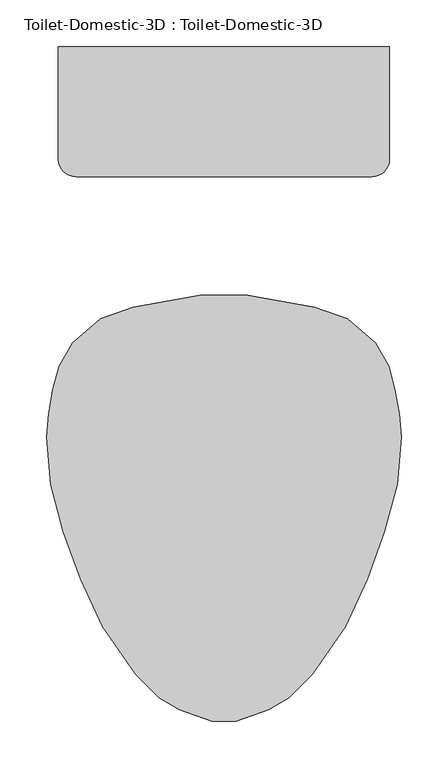
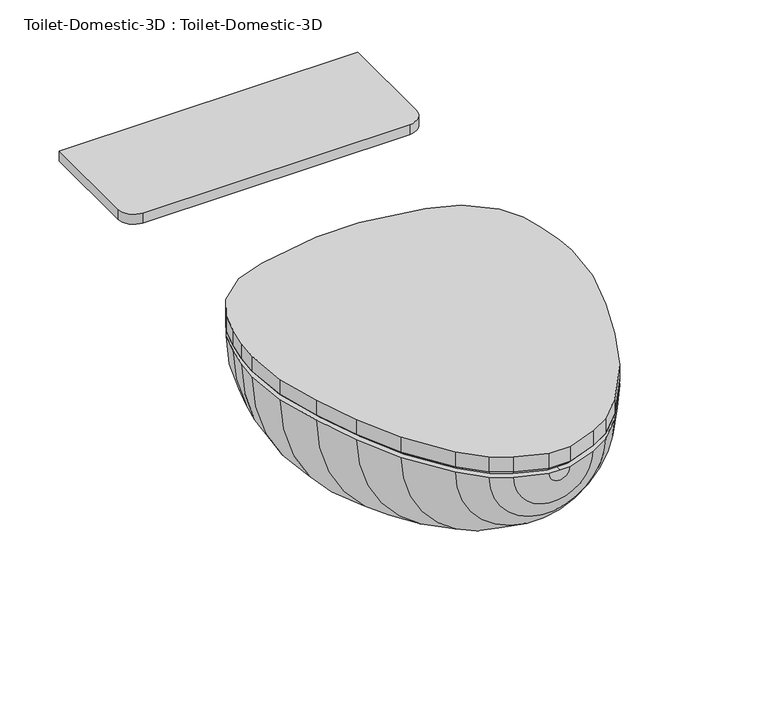
"""IFC4 building model written with IfcOpenShell, lengths in millimetres: flow terminal geometry, Toilet-Domestic-3D : Toilet-Domestic-3D."""

import ifcopenshell
import ifcopenshell.guid

model = None  # the IFC model being written
_history = None  # IfcOwnerHistory: only IFC2X3 demands one
_inside = {}  # id of a spatial element -> (the spatial element, [elements in it])
_under = {}  # id of a project, library or spatial element -> (it, [spatial elements below it])
_declared = {}  # id of a project -> (the project, [libraries it declares])
_typed = {}  # id of a type object -> (the type object, [elements of that type])
_made_of = {}  # id of a material, layer set ... -> (it, [elements and type objects made of it])


def new_model(schema):
    """Start an empty IFC model of exactly this schema.

    Asked for "IFC4X3", IfcOpenShell would pick the latest addendum, in which some entities
    have other attributes; the version numbers below select the first issue.
    IFC2X3 requires an IfcOwnerHistory on every rooted entity: one is made here for all.
    """
    global model, _history
    if schema == "IFC4X3":
        model = ifcopenshell.file(schema_version=(4, 3, 0, 0))
    else:
        model = ifcopenshell.file(schema=schema)
    _inside.clear()
    _under.clear()
    _declared.clear()
    _typed.clear()
    _made_of.clear()
    _history = None
    if model.schema == "IFC2X3":
        org = make("IfcOrganization", Name="unknown")
        user = make(
            "IfcPersonAndOrganization",
            ThePerson=make("IfcPerson", FamilyName="unknown"),
            TheOrganization=org,
        )
        app = make(
            "IfcApplication",
            ApplicationDeveloper=org,
            Version="unknown",
            ApplicationFullName="unknown",
            ApplicationIdentifier="unknown",
        )
        _history = make(
            "IfcOwnerHistory",
            OwningUser=user,
            OwningApplication=app,
            ChangeAction="ADDED",
            CreationDate=0,
        )
    return model


def make(cls, **values):
    """One entity of the class cls with the attributes given. An attribute that is None is left unset."""
    return model.create_entity(
        cls, **{name: value for name, value in values.items() if value is not None}
    )


def rooted(cls, **values):
    """An entity with a GlobalId (a new one), such as an element, a storey or a relation."""
    return make(cls, GlobalId=ifcopenshell.guid.new(), OwnerHistory=_history, **values)


def si_unit(unit_type, name, prefix=None):
    """IfcSIUnit, for example si_unit("LENGTHUNIT", "METRE", prefix="MILLI")."""
    return make("IfcSIUnit", UnitType=unit_type, Prefix=prefix, Name=name)


def assignment(units):
    """IfcUnitAssignment: the units of a project."""
    return None if units is None else make("IfcUnitAssignment", Units=units)


def point(xyz):
    """IfcCartesianPoint."""
    return None if xyz is None else make("IfcCartesianPoint", Coordinates=xyz)


def direction(xyz):
    """IfcDirection."""
    return None if xyz is None else make("IfcDirection", DirectionRatios=xyz)


def frame(location, z_axis=None, x_axis=None):
    """IfcAxis2Placement3D, a coordinate frame: its origin and axes. An axis left out is left unset."""
    return make(
        "IfcAxis2Placement3D",
        Location=point(location),
        Axis=direction(z_axis),
        RefDirection=direction(x_axis),
    )


def frame_2d(location, x_axis=None):
    """IfcAxis2Placement2D, a coordinate frame in the plane: its origin and x axis."""
    return make(
        "IfcAxis2Placement2D", Location=point(location), RefDirection=direction(x_axis)
    )


def origin():
    """The frame at (0, 0, 0) with its axes left unset."""
    return frame((0.0, 0.0, 0.0))


def place(relative_to, where):
    """IfcLocalPlacement: puts the frame where relative to a parent placement (None: the world)."""
    return make(
        "IfcLocalPlacement", PlacementRelTo=relative_to, RelativePlacement=where
    )


def context(
    kind, dimensions, precision=None, world=None, true_north=None, identifier=None
):
    """IfcGeometricRepresentationContext, for example the 3D "Model" context."""
    return make(
        "IfcGeometricRepresentationContext",
        ContextIdentifier=identifier,
        ContextType=kind,
        CoordinateSpaceDimension=dimensions,
        Precision=precision,
        WorldCoordinateSystem=world,
        TrueNorth=true_north,
    )


def project(units=None, contexts=None):
    """IfcProject with its units and contexts."""
    return rooted(
        "IfcProject",
        Name="project",
        RepresentationContexts=contexts,
        UnitsInContext=assignment(units),
    )


def spatial(cls, under=None, at=None, **own):
    """A site, building, storey or space (cls), placed at a placement, below another one or the project."""
    s = rooted(cls, ObjectPlacement=at, **own)
    if under is not None:
        _under.setdefault(under.id(), (under, []))[1].append(s)
    return s


def polyline(points):
    """IfcPolyline through the points."""
    return make("IfcPolyline", Points=[point(p) for p in points])


def circle_curve(where, radius):
    """IfcCircle in the frame where."""
    return make("IfcCircle", Position=where, Radius=radius)


def trimmed(basis, trim1, trim2, sense, master):
    """IfcTrimmedCurve: the piece of a basis curve between two trims."""
    return make(
        "IfcTrimmedCurve",
        BasisCurve=basis,
        Trim1=trim1,
        Trim2=trim2,
        SenseAgreement=sense,
        MasterRepresentation=master,
    )


def segment(curve, same_sense, transition):
    """IfcCompositeCurveSegment."""
    return make(
        "IfcCompositeCurveSegment",
        Transition=transition,
        SameSense=same_sense,
        ParentCurve=curve,
    )


def composite_curve(segments, self_intersect=None):
    """IfcCompositeCurve: segments joined end to end."""
    return make("IfcCompositeCurve", Segments=segments, SelfIntersect=self_intersect)


def outline(outer, holes=None, kind="AREA"):
    """IfcArbitraryClosedProfileDef: a profile drawn as a closed curve; with holes, ...WithVoids."""
    if holes is None:
        return make("IfcArbitraryClosedProfileDef", ProfileType=kind, OuterCurve=outer)
    return make(
        "IfcArbitraryProfileDefWithVoids",
        ProfileType=kind,
        OuterCurve=outer,
        InnerCurves=holes,
    )


def extrude(swept, where, along, depth):
    """IfcExtrudedAreaSolid: the profile swept, set in the frame where, extruded along a direction by depth."""
    return make(
        "IfcExtrudedAreaSolid",
        SweptArea=swept,
        Position=where,
        ExtrudedDirection=direction(along),
        Depth=depth,
    )


def faces_of(points, faces, orient=None, outer=None):
    """IfcFace entities. A face is a list of loops; a loop is a list of indices into points, from 0.

    orient and outer hold one flag for each loop. By default every Orientation is true, the
    first loop of a face is its IfcFaceOuterBound and the others are IfcFaceBound.
    """
    made = []
    for i, loops in enumerate(faces):
        bounds = []
        for j, loop in enumerate(loops):
            is_outer = j == 0 if outer is None else outer[i][j]
            bounds.append(
                make(
                    "IfcFaceOuterBound" if is_outer else "IfcFaceBound",
                    Bound=make("IfcPolyLoop", Polygon=[points[k] for k in loop]),
                    Orientation=True if orient is None else orient[i][j],
                )
            )
        made.append(make("IfcFace", Bounds=bounds))
    return made


def faceted_brep(points, faces, orient=None, outer=None, voids=None):
    """IfcFacetedBrep: a solid bounded by flat faces; with voids (closed shells), ...WithVoids."""
    shared = [point(p) for p in points]
    hull = make("IfcClosedShell", CfsFaces=faces_of(shared, faces, orient, outer))
    if voids is None:
        return make("IfcFacetedBrep", Outer=hull)
    return make(
        "IfcFacetedBrepWithVoids",
        Outer=hull,
        Voids=[
            make(cls, CfsFaces=faces_of(shared, fs, o, b)) for cls, fs, o, b in voids
        ],
    )


def shape(context_of_items, identifier, shape_type, items):
    """IfcShapeRepresentation: the items that make up one representation, for example the "Body"."""
    return make(
        "IfcShapeRepresentation",
        ContextOfItems=context_of_items,
        RepresentationIdentifier=identifier,
        RepresentationType=shape_type,
        Items=items,
    )


def source(mapping_origin, context_of_items, identifier, shape_type, items):
    """IfcRepresentationMap: a shape defined once, which mapped items show again and again."""
    return make(
        "IfcRepresentationMap",
        MappingOrigin=mapping_origin,
        MappedRepresentation=shape(context_of_items, identifier, shape_type, items),
    )


def transform(
    local_origin,
    x_axis=None,
    y_axis=None,
    z_axis=None,
    scale=None,
    scale2=None,
    scale3=None,
    uniform=True,
):
    """IfcCartesianTransformationOperator3D, or its non-uniform kind. x_axis, y_axis, z_axis: its Axis1, 2, 3."""
    if uniform:
        return make(
            "IfcCartesianTransformationOperator3D",
            Axis1=direction(x_axis),
            Axis2=direction(y_axis),
            LocalOrigin=point(local_origin),
            Scale=scale,
            Axis3=direction(z_axis),
        )
    return make(
        "IfcCartesianTransformationOperator3DnonUniform",
        Axis1=direction(x_axis),
        Axis2=direction(y_axis),
        LocalOrigin=point(local_origin),
        Scale=scale,
        Axis3=direction(z_axis),
        Scale2=scale2,
        Scale3=scale3,
    )


def mapped(mapping_source, mapping_target):
    """IfcMappedItem: shows the shape of a source again, moved by a transform."""
    return make(
        "IfcMappedItem", MappingSource=mapping_source, MappingTarget=mapping_target
    )


def made_of(thing, what):
    """Note that an element or type object is made of a material, layer set ...; save() writes the relation."""
    if what is not None:
        _made_of.setdefault(what.id(), (what, []))[1].append(thing)
    return thing


def element(
    cls,
    number,
    at=None,
    inside=None,
    cuts=None,
    type_object=None,
    material=None,
    context=None,
    identifier="Body",
    shape_type=None,
    held_by="IfcProductDefinitionShape",
    body=None,
    shapes=None,
    **own,
):
    """One element of the class cls, such as IfcWall. Its Tag is "e" and its number.

    at: its placement. inside: the storey or other place that contains it. cuts: it is an
    opening in that element (IfcRelVoidsElement). A single representation is given by context,
    identifier, shape_type and body (its items); several are given by shapes. held_by: the class
    of the entity that holds the representations. save() writes the other relations.
    """
    e = rooted(cls, Tag="e%d" % number, ObjectPlacement=at, **own)
    if body is not None:
        shapes = [shape(context, identifier, shape_type, body)]
    if shapes is not None:
        e.Representation = make(held_by, Representations=shapes)
    if inside is not None:
        _inside.setdefault(inside.id(), (inside, []))[1].append(e)
    if cuts is not None:
        rooted(
            "IfcRelVoidsElement", RelatingBuildingElement=cuts, RelatedOpeningElement=e
        )
    if type_object is not None:
        _typed.setdefault(type_object.id(), (type_object, []))[1].append(e)
    return made_of(e, material)


def aggregate(whole, parts):
    """IfcRelAggregates: a whole, such as a stair, and the parts it consists of."""
    return rooted("IfcRelAggregates", RelatingObject=whole, RelatedObjects=parts)


def save(model, path):
    """Write the relations noted so far, then the file.

    IfcRelAggregates (storeys below a building ...), IfcRelContainedInSpatialStructure (elements
    in a storey), IfcRelDefinesByType, IfcRelAssociatesMaterial and IfcRelDeclares: one each for
    every whole, place, type object, material and project.
    """
    for whole, parts in _under.values():
        aggregate(whole, parts)
    for where, things in _inside.values():
        rooted(
            "IfcRelContainedInSpatialStructure",
            RelatedElements=things,
            RelatingStructure=where,
        )
    for kind, things in _typed.values():
        rooted("IfcRelDefinesByType", RelatedObjects=things, RelatingType=kind)
    for what, things in _made_of.values():
        rooted("IfcRelAssociatesMaterial", RelatedObjects=things, RelatingMaterial=what)
    for by, libraries in _declared.values():
        rooted("IfcRelDeclares", RelatingContext=by, RelatedDefinitions=libraries)
    model.write(path)


def plane_surface(at):
    """IfcPlane: the flat surface through the origin of the frame at, square to its z axis."""
    return make("IfcPlane", Position=at)


def revolved_surface(curve, axis_point, axis_direction):
    """IfcSurfaceOfRevolution: the curve turned about the line through axis_point along axis_direction."""
    return make(
        "IfcSurfaceOfRevolution",
        SweptCurve=make("IfcArbitraryOpenProfileDef", ProfileType="CURVE", Curve=curve),
        AxisPosition=make("IfcAxis1Placement", Location=point(axis_point), Axis=direction(axis_direction)),
    )


def advanced_brep(points, edges, surfaces, faces):
    """IfcAdvancedBrep: a solid bounded by faces that lie on surfaces and meet in shared edges.

    An edge is (start, end): straight between two places in points (the first is 0);
    or (start, end, curve); or (start, end, curve, False) where it runs against its curve.
    A face is (place in surfaces, loops), or (place, loops, False) where it looks against
    its surface's normal. A loop lists edges by number (the first is 1), with a minus sign
    where the edge is run from its end to its start. The first loop is the outer one.
    """
    corners = [point(p) for p in points]
    vertices = [make("IfcVertexPoint", VertexGeometry=c) for c in corners]
    made = []
    for start, end, *more in edges:
        made.append(
            make(
                "IfcEdgeCurve",
                EdgeStart=vertices[start],
                EdgeEnd=vertices[end],
                EdgeGeometry=more[0] if more else make("IfcPolyline", Points=[corners[start], corners[end]]),
                SameSense=more[1] if len(more) > 1 else True,
            )
        )
    hull = []
    for where, loops, *sense in faces:
        bounds = []
        for j, loop in enumerate(loops):
            ring = [make("IfcOrientedEdge", EdgeElement=made[abs(k) - 1], Orientation=k > 0) for k in loop]
            bounds.append(
                make(
                    "IfcFaceOuterBound" if j == 0 else "IfcFaceBound",
                    Bound=make("IfcEdgeLoop", EdgeList=ring),
                    Orientation=True,
                )
            )
        hull.append(make("IfcAdvancedFace", Bounds=bounds, FaceSurface=surfaces[where], SameSense=sense[0] if sense else True))
    return make("IfcAdvancedBrep", Outer=make("IfcClosedShell", CfsFaces=hull))


def toilet_domestic_3d_toilet_domestic_3d_183bbd19(model_context):
    return source(origin(), model_context, "Body", "SolidModel", [
        advanced_brep(
        [(-25.4, 152.4, 361.95), (-97.4252791, 139.7, 361.95), (-132.3182423, 127.0, 361.95), (-162.5887836, 101.6, 361.95), (-176.9845865, 76.2, 361.95), (-183.790496, 50.8, 361.95), (-188.2862441, 25.3033453, 361.95), (-190.5, 0.0, 361.95), (-186.0724883, -50.6066907, 361.95), (-172.4088722, -101.6, 361.95), (-153.9191843, -152.4, 361.95), (-130.2307553, -203.2, 361.95), (-94.9900085, -254.0, 361.95), (-69.5900085, -279.4, 361.95), (-47.5929632, -292.1, 361.95), (-12.7, -304.8, 361.95), (0.0, -304.8, 361.95), (0.0, -284.592034, 361.95), (-12.5224565, -284.592034, 361.95), (-39.5113323, -274.7688865, 361.95), (-58.4178985, -263.8531754, 361.95), (-79.2146703, -243.0564036, 361.95), (-114.0255101, -192.8761202, 361.95), (-136.654021, -144.3491221, 361.95), (-154.575847, -95.1093097, 361.95), (-167.7238545, -46.0402777, 361.95), (-171.5645445, -2.1409906, 361.95), (-169.3087351, 23.6430284, 361.95), (-165.101298, 47.5045901, 361.95), (-159.5484355, 68.2281551, 361.95), (-146.1085923, 90.5605136, 361.95), (-121.9980886, 110.7916284, 361.95), (-94.1172813, 120.9394123, 361.95), (-22.0920022, 133.6394123, 361.95), (0.0, 133.6394123, 361.95), (0.0, 152.4, 361.95), (25.4, 152.4, 361.95), (22.0920022, 133.6394123, 361.95), (94.1172813, 120.9394123, 361.95), (121.9980886, 110.7916284, 361.95), (146.1085923, 90.5605136, 361.95), (159.5484355, 68.2281551, 361.95), (165.101298, 47.5045901, 361.95), (169.3087351, 23.6430284, 361.95), (171.5645445, -2.1409906, 361.95), (167.7238545, -46.0402777, 361.95), (154.575847, -95.1093097, 361.95), (136.654021, -144.3491221, 361.95), (114.0255101, -192.8761202, 361.95), (79.2146703, -243.0564036, 361.95), (58.4178985, -263.8531754, 361.95), (39.5113323, -274.7688865, 361.95), (12.5224565, -284.592034, 361.95), (12.7, -304.8, 361.95), (47.5929632, -292.1, 361.95), (69.5900085, -279.4, 361.95), (94.9900085, -254.0, 361.95), (130.2307553, -203.2, 361.95), (153.9191843, -152.4, 361.95), (172.4088722, -101.6, 361.95), (186.0724883, -50.6066907, 361.95), (190.5, 0.0, 361.95), (188.2862441, 25.3033453, 361.95), (183.790496, 50.8, 361.95), (176.9845865, 76.2, 361.95), (162.5887836, 101.6, 361.95), (132.3182423, 127.0, 361.95), (97.4252791, 139.7, 361.95)],
        [
            (0, 1),
            (1, 2),
            (2, 3),
            (3, 4),
            (4, 5),
            (5, 6),
            (6, 7),
            (7, 8),
            (8, 9),
            (9, 10),
            (10, 11),
            (11, 12),
            (12, 13),
            (13, 14),
            (14, 15),
            (15, 16),
            (16, 17),
            (17, 18),
            (18, 19),
            (19, 20),
            (20, 21),
            (21, 22),
            (22, 23),
            (23, 24),
            (24, 25),
            (25, 26),
            (26, 27),
            (27, 28),
            (28, 29),
            (29, 30),
            (30, 31),
            (31, 32),
            (32, 33),
            (33, 34),
            (34, 35),
            (35, 0),
            (36, 35),
            (34, 37),
            (37, 38),
            (38, 39),
            (39, 40),
            (40, 41),
            (41, 42),
            (42, 43),
            (43, 44),
            (44, 45),
            (45, 46),
            (46, 47),
            (47, 48),
            (48, 49),
            (49, 50),
            (50, 51),
            (51, 52),
            (52, 17),
            (16, 53),
            (53, 54),
            (54, 55),
            (55, 56),
            (56, 57),
            (57, 58),
            (58, 59),
            (59, 60),
            (60, 61),
            (61, 62),
            (62, 63),
            (63, 64),
            (64, 65),
            (65, 66),
            (66, 67),
            (67, 36),
            (67, 1, circle_curve(frame((0.0, 139.7, 361.95), z_axis=(0.0, 1.0, 0.0), x_axis=(-1.0, 0.0, 0.0)), 97.4252791)),
            (0, 36, circle_curve(frame((0.0, 152.4, 361.95), z_axis=(0.0, -1.0, 0.0), x_axis=(-1.0, 0.0, 0.0)), 25.4)),
            (66, 2, circle_curve(frame((0.0, 127.0, 361.95), z_axis=(0.0, 1.0, 0.0), x_axis=(-1.0, 0.0, 0.0)), 132.3182423)),
            (65, 3, circle_curve(frame((0.0, 101.6, 361.95), z_axis=(0.0, 1.0, 0.0), x_axis=(-1.0, 0.0, 0.0)), 162.5887836)),
            (64, 4, circle_curve(frame((0.0, 76.2, 361.95), z_axis=(0.0, 1.0, 0.0), x_axis=(-1.0, 0.0, 0.0)), 176.9845865)),
            (63, 5, circle_curve(frame((0.0, 50.8, 361.95), z_axis=(0.0, 1.0, 0.0), x_axis=(-1.0, 0.0, 0.0)), 183.790496)),
            (62, 6, circle_curve(frame((0.0, 25.3033453, 361.95), z_axis=(0.0, 1.0, 0.0), x_axis=(-1.0, 0.0, 0.0)), 188.2862441)),
            (61, 7, circle_curve(frame((0.0, 0.0, 361.95), z_axis=(0.0, 1.0, 0.0), x_axis=(-1.0, 0.0, 0.0)), 190.5)),
            (60, 8, circle_curve(frame((0.0, -50.6066907, 361.95), z_axis=(0.0, 1.0, 0.0), x_axis=(-1.0, 0.0, 0.0)), 186.0724883)),
            (59, 9, circle_curve(frame((0.0, -101.6, 361.95), z_axis=(0.0, 1.0, 0.0), x_axis=(-1.0, 0.0, 0.0)), 172.4088722)),
            (58, 10, circle_curve(frame((0.0, -152.4, 361.95), z_axis=(0.0, 1.0, 0.0), x_axis=(-1.0, 0.0, 0.0)), 153.9191843)),
            (57, 11, circle_curve(frame((0.0, -203.2, 361.95), z_axis=(0.0, 1.0, 0.0), x_axis=(-1.0, 0.0, 0.0)), 130.2307553)),
            (56, 12, circle_curve(frame((0.0, -254.0, 361.95), z_axis=(0.0, 1.0, 0.0), x_axis=(-1.0, 0.0, 0.0)), 94.9900085)),
            (55, 13, circle_curve(frame((0.0, -279.4, 361.95), z_axis=(0.0, 1.0, 0.0), x_axis=(-1.0, 0.0, 0.0)), 69.5900085)),
            (54, 14, circle_curve(frame((0.0, -292.1, 361.95), z_axis=(0.0, 1.0, 0.0), x_axis=(-1.0, 0.0, 0.0)), 47.5929632)),
            (53, 15, circle_curve(frame((0.0, -304.8, 361.95), z_axis=(0.0, 1.0, 0.0), x_axis=(-1.0, 0.0, 0.0)), 12.7)),
            (52, 18, circle_curve(frame((0.0, -284.592034, 361.95), z_axis=(0.0, 1.0, 0.0), x_axis=(-1.0, 0.0, 0.0)), 12.5224565)),
            (51, 19, circle_curve(frame((0.0, -274.7688865, 361.95), z_axis=(0.0, 1.0, 0.0), x_axis=(-1.0, 0.0, 0.0)), 39.5113323)),
            (50, 20, circle_curve(frame((0.0, -263.8531754, 361.95), z_axis=(0.0, 1.0, 0.0), x_axis=(-1.0, 0.0, 0.0)), 58.4178985)),
            (49, 21, circle_curve(frame((0.0, -243.0564036, 361.95), z_axis=(0.0, 1.0, 0.0), x_axis=(-1.0, 0.0, 0.0)), 79.2146703)),
            (48, 22, circle_curve(frame((0.0, -192.8761202, 361.95), z_axis=(0.0, 1.0, 0.0), x_axis=(-1.0, 0.0, 0.0)), 114.0255101)),
            (47, 23, circle_curve(frame((0.0, -144.3491221, 361.95), z_axis=(0.0, 1.0, 0.0), x_axis=(-1.0, 0.0, 0.0)), 136.654021)),
            (46, 24, circle_curve(frame((0.0, -95.1093097, 361.95), z_axis=(0.0, 1.0, 0.0), x_axis=(-1.0, 0.0, 0.0)), 154.575847)),
            (45, 25, circle_curve(frame((0.0, -46.0402777, 361.95), z_axis=(0.0, 1.0, 0.0), x_axis=(-1.0, 0.0, 0.0)), 167.7238545)),
            (44, 26, circle_curve(frame((0.0, -2.1409906, 361.95), z_axis=(0.0, 1.0, 0.0), x_axis=(-1.0, 0.0, 0.0)), 171.5645445)),
            (43, 27, circle_curve(frame((0.0, 23.6430284, 361.95), z_axis=(0.0, 1.0, 0.0), x_axis=(-1.0, 0.0, 0.0)), 169.3087351)),
            (42, 28, circle_curve(frame((0.0, 47.5045901, 361.95), z_axis=(0.0, 1.0, 0.0), x_axis=(-1.0, 0.0, 0.0)), 165.101298)),
            (41, 29, circle_curve(frame((0.0, 68.2281551, 361.95), z_axis=(0.0, 1.0, 0.0), x_axis=(-1.0, 0.0, 0.0)), 159.5484355)),
            (40, 30, circle_curve(frame((0.0, 90.5605136, 361.95), z_axis=(0.0, 1.0, 0.0), x_axis=(-1.0, 0.0, 0.0)), 146.1085923)),
            (39, 31, circle_curve(frame((0.0, 110.7916284, 361.95), z_axis=(0.0, 1.0, 0.0), x_axis=(-1.0, 0.0, 0.0)), 121.9980886)),
            (38, 32, circle_curve(frame((0.0, 120.9394123, 361.95), z_axis=(0.0, 1.0, 0.0), x_axis=(-1.0, 0.0, 0.0)), 94.1172813)),
            (37, 33, circle_curve(frame((0.0, 133.6394123, 361.95), z_axis=(0.0, 1.0, 0.0), x_axis=(-1.0, 0.0, 0.0)), 22.0920022)),
        ],
        [
            plane_surface(frame((0.0, 175.1599017, 361.95), z_axis=(0.0, 0.0, 1.0), x_axis=(-1.0, 0.0, 0.0))),
            plane_surface(frame((0.0, 175.1599017, 361.95), z_axis=(0.0, 0.0, 1.0), x_axis=(1.0, 0.0, 0.0))),
            revolved_surface(polyline([(-25.4, 152.4, 361.95), (-97.4252791, 139.7, 361.95)]), (0.0, 175.1599017, 361.95), (0.0, -1.0, 0.0)),
            revolved_surface(polyline([(-97.4252791, 139.7, 361.95), (-132.3182423, 127.0, 361.95)]), (0.0, 175.1599017, 361.95), (0.0, -1.0, 0.0)),
            revolved_surface(polyline([(-132.3182423, 127.0, 361.95), (-162.5887836, 101.6, 361.95)]), (0.0, 175.1599017, 361.95), (0.0, -1.0, 0.0)),
            revolved_surface(polyline([(-162.5887836, 101.6, 361.95), (-176.9845865, 76.2, 361.95)]), (0.0, 175.1599017, 361.95), (0.0, -1.0, 0.0)),
            revolved_surface(polyline([(-176.9845865, 76.2, 361.95), (-183.790496, 50.8, 361.95)]), (0.0, 175.1599017, 361.95), (0.0, -1.0, 0.0)),
            revolved_surface(polyline([(-183.790496, 50.8, 361.95), (-188.2862441, 25.3033453, 361.95)]), (0.0, 175.1599017, 361.95), (0.0, -1.0, 0.0)),
            revolved_surface(polyline([(-188.2862441, 25.3033453, 361.95), (-190.5, 0.0, 361.95)]), (0.0, 175.1599017, 361.95), (0.0, -1.0, 0.0)),
            revolved_surface(polyline([(-190.5, 0.0, 361.95), (-186.0724883, -50.6066907, 361.95)]), (0.0, 175.1599017, 361.95), (0.0, -1.0, 0.0)),
            revolved_surface(polyline([(-186.0724883, -50.6066907, 361.95), (-172.4088722, -101.6, 361.95)]), (0.0, 175.1599017, 361.95), (0.0, -1.0, 0.0)),
            revolved_surface(polyline([(-172.4088722, -101.6, 361.95), (-153.9191843, -152.4, 361.95)]), (0.0, 175.1599017, 361.95), (0.0, -1.0, 0.0)),
            revolved_surface(polyline([(-153.9191843, -152.4, 361.95), (-130.2307553, -203.2, 361.95)]), (0.0, 175.1599017, 361.95), (0.0, -1.0, 0.0)),
            revolved_surface(polyline([(-130.2307553, -203.2, 361.95), (-94.9900085, -254.0, 361.95)]), (0.0, 175.1599017, 361.95), (0.0, -1.0, 0.0)),
            revolved_surface(polyline([(-94.9900085, -254.0, 361.95), (-69.5900085, -279.4, 361.95)]), (0.0, 175.1599017, 361.95), (0.0, -1.0, 0.0)),
            revolved_surface(polyline([(-69.5900085, -279.4, 361.95), (-47.5929632, -292.1, 361.95)]), (0.0, 175.1599017, 361.95), (0.0, -1.0, 0.0)),
            revolved_surface(polyline([(-47.5929632, -292.1, 361.95), (-12.7, -304.8, 361.95)]), (0.0, 175.1599017, 361.95), (0.0, -1.0, 0.0)),
            plane_surface(frame((0.0, -304.8, 361.95), z_axis=(0.0, -1.0, 0.0), x_axis=(-1.0, 0.0, 0.0))),
            plane_surface(frame((0.0, -284.592034, 361.95), z_axis=(0.0, 1.0, 0.0), x_axis=(-1.0, 0.0, 0.0))),
            revolved_surface(polyline([(-12.5224565, -284.592034, 361.95), (-39.5113323, -274.7688865, 361.95)]), (0.0, 175.1599017, 361.95), (0.0, -1.0, 0.0)),
            revolved_surface(polyline([(-39.5113323, -274.7688865, 361.95), (-58.4178985, -263.8531754, 361.95)]), (0.0, 175.1599017, 361.95), (0.0, -1.0, 0.0)),
            revolved_surface(polyline([(-58.4178985, -263.8531754, 361.95), (-79.2146703, -243.0564036, 361.95)]), (0.0, 175.1599017, 361.95), (0.0, -1.0, 0.0)),
            revolved_surface(polyline([(-79.2146703, -243.0564036, 361.95), (-114.0255101, -192.8761202, 361.95)]), (0.0, 175.1599017, 361.95), (0.0, -1.0, 0.0)),
            revolved_surface(polyline([(-114.0255101, -192.8761202, 361.95), (-136.654021, -144.3491221, 361.95)]), (0.0, 175.1599017, 361.95), (0.0, -1.0, 0.0)),
            revolved_surface(polyline([(-136.654021, -144.3491221, 361.95), (-154.575847, -95.1093097, 361.95)]), (0.0, 175.1599017, 361.95), (0.0, -1.0, 0.0)),
            revolved_surface(polyline([(-154.575847, -95.1093097, 361.95), (-167.7238545, -46.0402777, 361.95)]), (0.0, 175.1599017, 361.95), (0.0, -1.0, 0.0)),
            revolved_surface(polyline([(-167.7238545, -46.0402777, 361.95), (-171.5645445, -2.1409906, 361.95)]), (0.0, 175.1599017, 361.95), (0.0, -1.0, 0.0)),
            revolved_surface(polyline([(-171.5645445, -2.1409906, 361.95), (-169.3087351, 23.6430284, 361.95)]), (0.0, 175.1599017, 361.95), (0.0, -1.0, 0.0)),
            revolved_surface(polyline([(-169.3087351, 23.6430284, 361.95), (-165.101298, 47.5045901, 361.95)]), (0.0, 175.1599017, 361.95), (0.0, -1.0, 0.0)),
            revolved_surface(polyline([(-165.101298, 47.5045901, 361.95), (-159.5484355, 68.2281551, 361.95)]), (0.0, 175.1599017, 361.95), (0.0, -1.0, 0.0)),
            revolved_surface(polyline([(-159.5484355, 68.2281551, 361.95), (-146.1085923, 90.5605136, 361.95)]), (0.0, 175.1599017, 361.95), (0.0, -1.0, 0.0)),
            revolved_surface(polyline([(-146.1085923, 90.5605136, 361.95), (-121.9980886, 110.7916284, 361.95)]), (0.0, 175.1599017, 361.95), (0.0, -1.0, 0.0)),
            revolved_surface(polyline([(-121.9980886, 110.7916284, 361.95), (-94.1172813, 120.9394123, 361.95)]), (0.0, 175.1599017, 361.95), (0.0, -1.0, 0.0)),
            revolved_surface(polyline([(-94.1172813, 120.9394123, 361.95), (-22.0920022, 133.6394123, 361.95)]), (0.0, 175.1599017, 361.95), (0.0, -1.0, 0.0)),
            plane_surface(frame((0.0, 133.6394123, 361.95), z_axis=(0.0, -1.0, 0.0), x_axis=(-1.0, 0.0, 0.0))),
            plane_surface(frame((0.0, 152.4, 361.95), z_axis=(0.0, 1.0, 0.0), x_axis=(-1.0, 0.0, 0.0))),
        ],
        [
            (0, [[1, 2, 3, 4, 5, 6, 7, 8, 9, 10, 11, 12, 13, 14, 15, 16, 17, 18, 19, 20, 21, 22, 23, 24, 25, 26, 27, 28, 29, 30, 31, 32, 33, 34, 35, 36]]),
            (1, [[37, -35, 38, 39, 40, 41, 42, 43, 44, 45, 46, 47, 48, 49, 50, 51, 52, 53, 54, -17, 55, 56, 57, 58, 59, 60, 61, 62, 63, 64, 65, 66, 67, 68, 69, 70]]),
            (2, [[71, -1, 72, -70]]),
            (3, [[73, -2, -71, -69]]),
            (4, [[74, -3, -73, -68]]),
            (5, [[75, -4, -74, -67]]),
            (6, [[76, -5, -75, -66]]),
            (7, [[77, -6, -76, -65]]),
            (8, [[78, -7, -77, -64]]),
            (9, [[79, -8, -78, -63]]),
            (10, [[80, -9, -79, -62]]),
            (11, [[81, -10, -80, -61]]),
            (12, [[82, -11, -81, -60]]),
            (13, [[83, -12, -82, -59]]),
            (14, [[84, -13, -83, -58]]),
            (15, [[85, -14, -84, -57]]),
            (16, [[86, -15, -85, -56]]),
            (17, [[-16, -86, -55]]),
            (18, [[87, -18, -54]]),
            (19, [[88, -19, -87, -53]]),
            (20, [[89, -20, -88, -52]]),
            (21, [[90, -21, -89, -51]]),
            (22, [[91, -22, -90, -50]]),
            (23, [[92, -23, -91, -49]]),
            (24, [[93, -24, -92, -48]]),
            (25, [[94, -25, -93, -47]]),
            (26, [[95, -26, -94, -46]]),
            (27, [[96, -27, -95, -45]]),
            (28, [[97, -28, -96, -44]]),
            (29, [[98, -29, -97, -43]]),
            (30, [[99, -30, -98, -42]]),
            (31, [[100, -31, -99, -41]]),
            (32, [[101, -32, -100, -40]]),
            (33, [[102, -33, -101, -39]]),
            (34, [[-34, -102, -38]]),
            (35, [[-72, -36, -37]]),
        ],
    ),
        faceted_brep([(-97.4252791, 139.7, 368.3), (-132.3182423, 127.0, 368.3), (-162.5887836, 101.6, 368.3), (-176.9845865, 76.2, 368.3), (-183.790496, 50.8, 368.3), (-188.2862441, 25.3033453, 368.3), (-190.5, 0.0, 368.3), (-186.0724883, -50.6066907, 368.3), (-172.4088722, -101.6, 368.3), (-153.9191843, -152.4, 368.3), (-130.2307553, -203.2, 368.3), (-94.9900085, -254.0, 368.3), (-69.5900085, -279.4, 368.3), (-47.5929632, -292.1, 368.3), (-12.7, -304.8, 368.3), (12.7, -304.8, 368.3), (47.5929632, -292.1, 368.3), (69.5900085, -279.4, 368.3), (94.9900085, -254.0, 368.3), (130.2307553, -203.2, 368.3), (153.9191843, -152.4, 368.3), (172.4088722, -101.6, 368.3), (186.0724883, -50.6066907, 368.3), (190.5, 0.0, 368.3), (188.2862441, 25.3033453, 368.3), (183.790496, 50.8, 368.3), (176.9845865, 76.2, 368.3), (162.5887836, 101.6, 368.3), (132.3182423, 127.0, 368.3), (97.4252791, 139.7, 368.3), (25.4, 152.4, 368.3), (-25.4, 152.4, 368.3), (-95.7755003, 133.5429415, 361.95), (-24.844447, 146.05, 361.95), (24.844447, 146.05, 361.95), (95.7755003, 133.5429415, 361.95), (129.0942628, 121.4159037, 361.95), (157.6293435, 97.472128, 361.95), (171.060664, 73.773864, 361.95), (177.5851102, 49.4242991, 361.95), (181.9845715, 24.4737144, 361.95), (184.125744, 0.0, 361.95), (179.7950716, -49.4998127, 361.95), (166.347, -99.688699, 361.95), (148.0469602, -149.9676451, 361.95), (124.7045808, -200.0255393, 361.95), (90.0971582, -249.9125941, 361.95), (65.691017, -274.3187354, 361.95), (44.8990862, -286.3229622, 361.95), (11.5803237, -298.45, 361.95), (-11.5803237, -298.45, 361.95), (-44.8990862, -286.3229622, 361.95), (-65.691017, -274.3187354, 361.95), (-90.0971582, -249.9125941, 361.95), (-124.7045808, -200.0255393, 361.95), (-148.0469602, -149.9676451, 361.95), (-166.347, -99.688699, 361.95), (-179.7950716, -49.4998127, 361.95), (-184.125744, 0.0, 361.95), (-181.9845715, 24.4737144, 361.95), (-177.5851102, 49.4242991, 361.95), (-171.060664, 73.773864, 361.95), (-157.6293435, 97.472128, 361.95), (-129.0942628, 121.4159037, 361.95)], [[[0, 1, 2, 3, 4, 5, 6, 7, 8, 9, 10, 11, 12, 13, 14, 15, 16, 17, 18, 19, 20, 21, 22, 23, 24, 25, 26, 27, 28, 29, 30, 31]], [[32, 33, 34, 35, 36, 37, 38, 39, 40, 41, 42, 43, 44, 45, 46, 47, 48, 49, 50, 51, 52, 53, 54, 55, 56, 57, 58, 59, 60, 61, 62, 63]], [[32, 63, 1, 0]], [[63, 62, 2, 1]], [[62, 61, 3, 2]], [[61, 60, 4, 3]], [[60, 59, 5, 4]], [[59, 58, 6, 5]], [[58, 57, 7, 6]], [[57, 56, 8, 7]], [[56, 55, 9, 8]], [[55, 54, 10, 9]], [[54, 53, 11, 10]], [[53, 52, 12, 11]], [[52, 51, 13, 12]], [[51, 50, 14, 13]], [[50, 49, 15, 14]], [[49, 48, 16, 15]], [[48, 47, 17, 16]], [[47, 46, 18, 17]], [[46, 45, 19, 18]], [[45, 44, 20, 19]], [[44, 43, 21, 20]], [[43, 42, 22, 21]], [[42, 41, 23, 22]], [[41, 40, 24, 23]], [[40, 39, 25, 24]], [[39, 38, 26, 25]], [[38, 37, 27, 26]], [[37, 36, 28, 27]], [[36, 35, 29, 28]], [[35, 34, 30, 29]], [[34, 33, 31, 30]], [[33, 32, 0, 31]]]),
        extrude(outline(composite_curve([segment(polyline([(177.8, 419.1), (177.8, 298.45)]), True, "CONTINUOUS"), segment(trimmed(circle_curve(frame_2d((158.75, 298.45)), 19.05), [point((177.8, 298.45))], [point((158.75, 279.4))], False, "CARTESIAN"), True, "CONTINUOUS"), segment(polyline([(158.75, 279.4), (-158.75, 279.4)]), True, "CONTINUOUS"), segment(trimmed(circle_curve(frame_2d((-158.75, 298.45)), 19.05), [point((-158.75, 279.4))], [point((-177.8, 298.45))], False, "CARTESIAN"), True, "CONTINUOUS"), segment(polyline([(-177.8, 298.45), (-177.8, 419.1), (177.8, 419.1)]), True, "CONTINUOUS")], self_intersect=False)), frame((0.0, 0.0, 374.65), z_axis=(0.0, 0.0, 1.0), x_axis=(1.0, 0.0, 0.0)), (0.0, 0.0, 1.0), 12.5681453),
        extrude(outline(polyline([(-162.5887836, 101.6), (-132.3182423, 127.0), (-97.4252791, 139.7), (-25.4, 152.4), (25.4, 152.4), (97.4252791, 139.7), (132.3182423, 127.0), (162.5887836, 101.6), (176.9845865, 76.2), (183.790496, 50.8), (188.2862441, 25.3033453), (190.5, 0.0), (186.0724883, -50.6066907), (172.4088722, -101.6), (153.9191843, -152.4), (130.2307553, -203.2), (94.9900085, -254.0), (69.5900085, -279.4), (47.5929632, -292.1), (12.7, -304.8), (-12.7, -304.8), (-47.5929632, -292.1), (-69.5900085, -279.4), (-94.9900085, -254.0), (-130.2307553, -203.2), (-153.9191843, -152.4), (-172.4088722, -101.6), (-186.0724883, -50.6066907), (-190.5, 0.0), (-188.2862441, 25.3033453), (-183.790496, 50.8), (-176.9845865, 76.2), (-162.5887836, 101.6)])), frame((0.0, 0.0, 368.3), z_axis=(0.0, 0.0, 1.0), x_axis=(1.0, 0.0, 0.0)), (0.0, 0.0, 1.0), 19.05),
    ])


if __name__ == "__main__":
    model = new_model("IFC4")
    model_context = context("Model", 3, world=origin())
    ifc_project = project(units=[si_unit("LENGTHUNIT", "METRE", prefix="MILLI")], contexts=[model_context])
    site = spatial("IfcSite", under=ifc_project)
    building = spatial("IfcBuilding", under=site)
    placement = place(None, origin())
    toilet_domestic_3d_toilet_domestic_3d_shape = toilet_domestic_3d_toilet_domestic_3d_183bbd19(model_context)
    element("IfcFlowTerminal", 1, ObjectType="Toilet-Domestic-3D : Toilet-Domestic-3D", at=placement, inside=building, context=model_context, shape_type="MappedRepresentation", body=[
        mapped(toilet_domestic_3d_toilet_domestic_3d_shape, transform((0.0, 0.0, 0.0), x_axis=(1.0, 0.0, 0.0), y_axis=(0.0, 1.0, 0.0), z_axis=(0.0, 0.0, 1.0))),
    ])
    save(model, "model.ifc")

# Revit data of these elements
# Type "Toilet-Domestic-3D : Toilet-Domestic-3D"
#   Assembly Code = "D2010110"
#   Toilet - Bowl/Basin Material = Porcelain, Linen
#   Toilet - Seat Material = Laminate, Linen, Matte
# Element 1 (IfcFlowTerminal, "Toilet-Domestic-3D : Toilet-Domestic-3D")
#   Materials on its faces: "Porcelain, Linen", "Laminate, Linen, Matte"
# Materials
#   "Porcelain, Linen": class "Ceramic", colour RGB 249 239 230, transparency 0, Description = "Porcelain, linen", Cost = 0
#   "Laminate, Linen, Matte": class "Plastic", colour RGB 249 239 230, transparency 0, Description = "Plastic Laminate - Linen, Matte", Cost = 0
